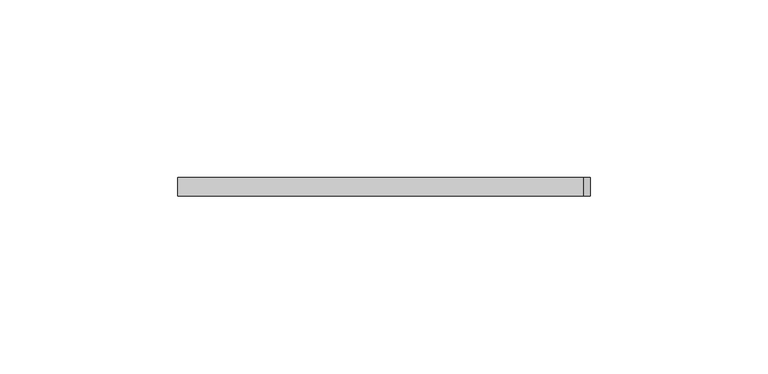
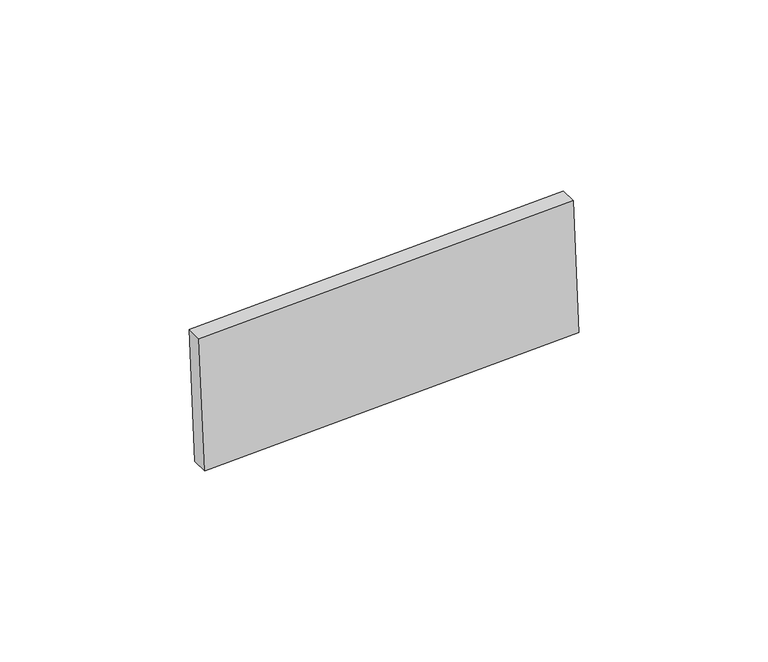
"""IFC4 building model written with IfcOpenShell, lengths in millimetres: proxy geometry, Inner panel:Inner panel:1:Inner panel:1 : Inner panel:Inner panel:300324:2:Inner panel:1:Inner panel:1 : Inner panel:Inner panel:300324:2 : Inner panel:Inner panel:1:Inner panel:1 : Inner panel:Inner panel:300324:300043:148 : Inner panel:Inner panel:1:Inner panel:1 : Inner panel:Inner panel:300324:2:Inner panel:1:Inner panel:1 : Inner panel:Inner panel:300324:2 : Inner panel:Inner panel:1:Inner panel:1 : Inner panel:Inner panel:300324:300043:308120."""

from ifc_helpers import new_model, si_unit, frame, origin, place, context, project, spatial, polyline, outline, extrude, source, transform, mapped, element, save


def generic_models_ca14916e(model_context):
    return source(origin(), model_context, "Body", "SweptSolid", [
        extrude(outline(polyline([(0.0, -114.3), (0.0, 0.0), (5.2138089, 0.0), (5.2138089, -114.3), (0.0, -114.3)])), frame((558340.6073057, -578534.9848948, 3867.9996071), z_axis=(-0.04163054471216399, 0.0, 0.9991330730923527), x_axis=(0.0, -1.0, 0.0)), (0.0, 0.0, 1.0), 43.2233908),
    ])


if __name__ == "__main__":
    model = new_model("IFC4")
    model_context = context("Model", 3, world=origin())
    ifc_project = project(units=[si_unit("LENGTHUNIT", "METRE", prefix="MILLI")], contexts=[model_context])
    site = spatial("IfcSite", under=ifc_project)
    building = spatial("IfcBuilding", under=site)
    placement = place(None, origin())
    generic_models_shape = generic_models_ca14916e(model_context)
    element("IfcBuildingElementProxy", 1, Name="Inner panel:Inner panel:1:Inner panel:1 : Inner panel:Inner panel:300324:2:Inner panel:1:Inner panel:1 : Inner panel:Inner panel:300324:2 : Inner panel:Inner panel:1:Inner panel:1 : Inner panel:Inner panel:300324:300043:148 : Inner panel:Inner panel:1:Inner panel:1 : Inner panel:Inner panel:300324:2:Inner panel:1:Inner panel:1 : Inner panel:Inner panel:300324:2 : Inner panel:Inner panel:1:Inner panel:1 : Inner panel:Inner panel:300324:300043:308120", ObjectType="Inner panel:Inner panel:1:Inner panel:1 : Inner panel:Inner panel:300324:2:Inner panel:1:Inner panel:1 : Inner panel:Inner panel:300324:2 : Inner panel:Inner panel:1:Inner panel:1 : Inner panel:Inner panel:300324:300043:148 : Inner panel:Inner panel:1:Inner panel:1 : Inner panel:Inner panel:300324:2:Inner panel:1:Inner panel:1 : Inner panel:Inner panel:300324:2 : Inner panel:Inner panel:1:Inner panel:1 : Inner panel:Inner panel:300324:300043:308120", at=placement, inside=building, context=model_context, shape_type="MappedRepresentation", body=[
        mapped(generic_models_shape, transform((0.0, 0.0, 0.0), x_axis=(1.0, 0.0, 0.0), y_axis=(0.0, 1.0, 0.0), z_axis=(0.0, 0.0, 1.0))),
    ])
    save(model, "model.ifc")

# Revit data of these elements
# Type "Inner panel:Inner panel:1:Inner panel:1 : Inner panel:Inner panel:300324:2:Inner panel:1:Inner panel:1 : Inner panel:Inner panel:300324:2 : Inner panel:Inner panel:1:Inner panel:1 : Inner panel:Inner panel:300324:300043:148 : Inner panel:Inner panel:1:Inner panel:1 : Inner panel:Inner panel:300324:2:Inner panel:1:Inner panel:1 : Inner panel:Inner panel:300324:2 : Inner panel:Inner panel:1:Inner panel:1 : Inner panel:Inner panel:300324:300043:308120"
#   NameOverride = "Inner panel:Inner panel:1:Inner panel:1 : Inner panel:Inner panel:300324:2:Inner panel:1:Inner panel:1 : Inner panel:Inner panel:300324:2 : Inner panel:Inner panel:1:Inner panel:1 : Inner panel:Inner panel:300324:300043:308120"
#   ObjectTypeOverride = "Inner panel:1:Inner panel:1 : Inner panel:Inner panel:300324:2 : Inner panel:Inner panel:1:Inner panel:1 : Inner panel:Inner panel:300324:300043"
#   Reference = "Inner panel"
#   Tag = "308120"
# Element 1 (IfcBuildingElementProxy, "Inner panel:Inner panel:1:Inner panel:1 : Inner panel:Inner panel:300324:2:Inner panel:1:Inner panel:1 : Inner panel:Inner panel:300324:2 : Inner panel:Inner panel:1:Inner panel:1 : Inner panel:Inner panel:300324:300043:148 : Inner panel:Inner panel:1:Inner panel:1 : Inner panel:Inner panel:300324:2:Inner panel:1:Inner panel:1 : Inner panel:Inner panel:300324:2 : Inner panel:Inner panel:1:Inner panel:1 : Inner panel:Inner panel:300324:300043:308120")
#   Materials on its faces: "SLIDING CLIP"
# Materials
#   "SLIDING CLIP": class "Generic", colour RGB 120 120 120, transparency 0, Cost = 0
